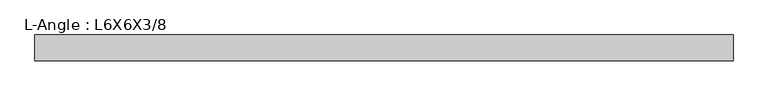
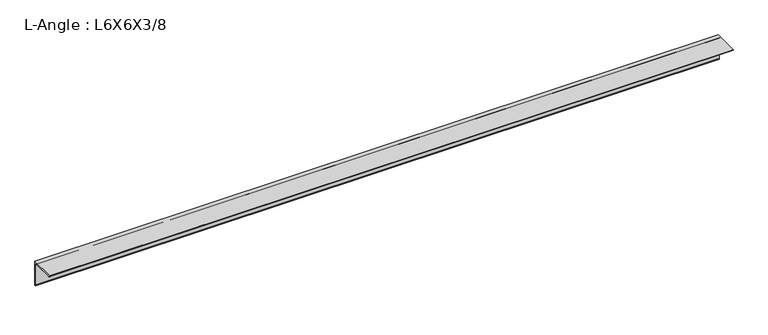
"""IFC4 building model written with IfcOpenShell, lengths in millimetres: member geometry, L-Angle : L6X6X3/8."""

from ifc_helpers import new_model, si_unit, point, frame, frame_2d, origin, place, context, project, spatial, polyline, circle_curve, trimmed, segment, composite_curve, outline, extrude, source, transform, mapped, element, save


def l_angle_l6x6x3_8_1e5b70da(model_context):
    return source(origin(), model_context, "Body", "SweptSolid", [
        extrude(outline(composite_curve([segment(polyline([(41.148, 41.148), (41.148, -111.252)]), True, "CONTINUOUS"), segment(trimmed(circle_curve(frame_2d((41.148, -101.727)), 9.525), [point((41.148, -111.252))], [point((31.623, -101.727))], False, "CARTESIAN"), True, "CONTINUOUS"), segment(polyline([(31.623, -101.727), (31.623, 22.098)]), True, "CONTINUOUS"), segment(trimmed(circle_curve(frame_2d((22.098, 22.098)), 9.525), [point((31.623, 22.098))], [point((22.098, 31.623))], True, "CARTESIAN"), True, "CONTINUOUS"), segment(polyline([(22.098, 31.623), (-101.727, 31.623)]), True, "CONTINUOUS"), segment(trimmed(circle_curve(frame_2d((-101.727, 41.148)), 9.525), [point((-101.727, 31.623))], [point((-111.252, 41.148))], False, "CARTESIAN"), True, "CONTINUOUS"), segment(polyline([(-111.252, 41.148), (41.148, 41.148)]), True, "CONTINUOUS")], self_intersect=False)), frame((-2053.4214347, 0.0, 0.0), z_axis=(1.0, 0.0, 0.0), x_axis=(0.0, 1.0, 0.0)), (0.0, 0.0, 1.0), 4092.1699392),
    ])


if __name__ == "__main__":
    model = new_model("IFC4")
    model_context = context("Model", 3, world=origin())
    ifc_project = project(units=[si_unit("LENGTHUNIT", "METRE", prefix="MILLI")], contexts=[model_context])
    site = spatial("IfcSite", under=ifc_project)
    building = spatial("IfcBuilding", under=site)
    placement = place(None, origin())
    l_angle_l6x6x3_8_shape = l_angle_l6x6x3_8_1e5b70da(model_context)
    element("IfcMember", 1, ObjectType="L-Angle : L6X6X3/8", at=placement, inside=building, context=model_context, shape_type="MappedRepresentation", body=[
        mapped(l_angle_l6x6x3_8_shape, transform((0.0, 0.0, 0.0), x_axis=(1.0, 0.0, 0.0), y_axis=(0.0, 1.0, 0.0), z_axis=(0.0, 0.0, 1.0))),
    ])
    save(model, "model.ifc")

# Revit data of these elements
# Type "L-Angle : L6X6X3/8"
#   Assembly Code = "B10"
#   k = 0' - 0 7/8"
#   W = 14.9
#   Length [instance default] = 5' - 0"
#   b = 0' - 6"
#   d = 0' - 6"
#   t = 0' - 0 3/8"
#   x = 0' - 1.62"
#   y = 0' - 1.62"
#   A = 0.0304167 SF
#   Structural Material [instance default] = Steel ASTM A36
# Element 1 (IfcMember, "L-Angle : L6X6X3/8")
#   Materials on its faces: "Steel ASTM A36"
# Materials
#   "Steel ASTM A36": class "Metal", colour RGB 199 199 199, transparency 0, Description = "Structural steel, ASTM A36 Grade B, mill finish", Cost = 0
